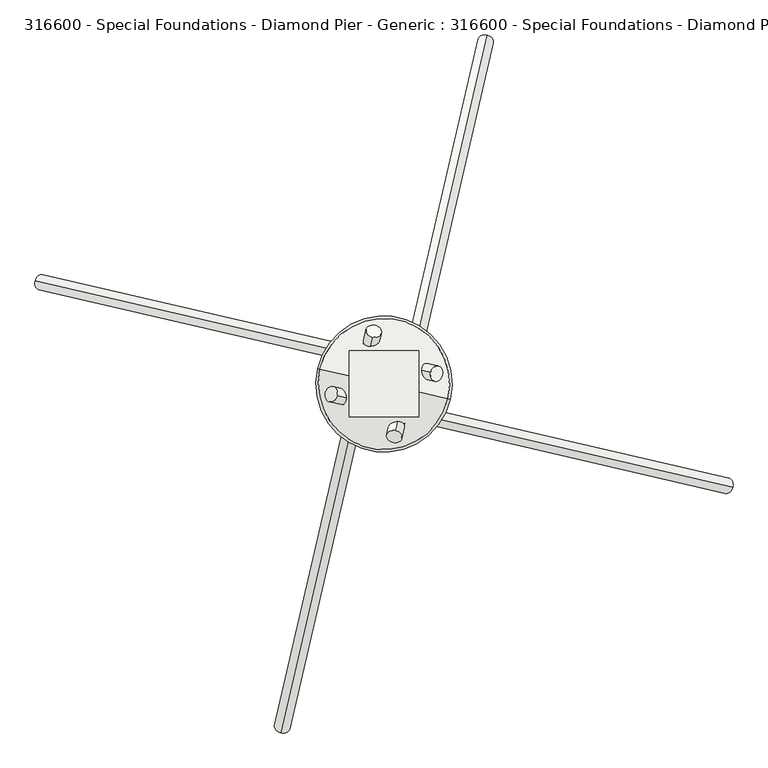
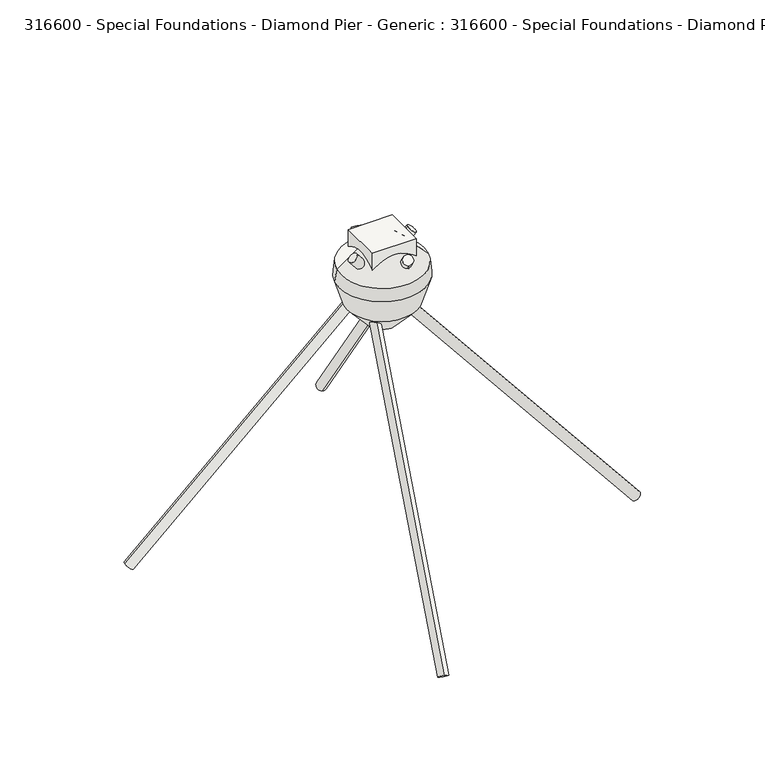
"""IFC4 building model written with IfcOpenShell, lengths in millimetres: slab geometry, 316600 - Special Foundations - Diamond Pier - Generic : 316600 - Special Foundations - Diamond Pier - Generic."""

from ifc_helpers import new_model, si_unit, point, frame, frame_2d, origin, place, context, project, spatial, polyline, circle_curve, trimmed, segment, composite_curve, outline, extrude, source, transform, mapped, element, save
from ifc_brep_helpers import plane_surface, revolved_surface, advanced_brep


def slab_316600_special_foundations_diamond_pier_generic_316600_ae65de88(model_context):
    return source(origin(), model_context, "Body", "SolidModel", [
        extrude(outline(composite_curve([segment(trimmed(circle_curve(frame_2d((1e-07, -15.875)), 15.875), [point((1e-07, -31.7500001))], [point((0.0, 0.0))], False, "CARTESIAN"), True, "CONTINUOUS"), segment(trimmed(circle_curve(frame_2d((1e-07, -15.875)), 15.875), [point((0.0, 0.0))], [point((1e-07, -31.7500001))], False, "CARTESIAN"), True, "CONTINUOUS")], self_intersect=False)), frame((-207.7929333, -703.2724242, -991.3584593), z_axis=(0.14520854647133766, 0.628002114484006, 0.7645441924671841), x_axis=(-0.9742942350214497, 0.2252792569322976, 0.0)), (0.0, 0.0, 1.0), 1270.0),
        extrude(outline(composite_curve([segment(trimmed(circle_curve(frame_2d((1e-07, -15.875)), 15.875), [point((1e-07, -31.7500001))], [point((0.0, 0.0))], False, "CARTESIAN"), True, "CONTINUOUS"), segment(trimmed(circle_curve(frame_2d((1e-07, -15.875)), 15.875), [point((0.0, 0.0))], [point((1e-07, -31.7500001))], False, "CARTESIAN"), True, "CONTINUOUS")], self_intersect=False)), frame((-703.2724242, 207.7929333, -991.3584593), z_axis=(0.6280021144840067, -0.14520854647133485, 0.7645441924671843), x_axis=(0.22527925693229323, 0.9742942350214507, 0.0)), (0.0, 0.0, 1.0), 1270.0),
        extrude(outline(composite_curve([segment(trimmed(circle_curve(frame_2d((1e-07, -15.875)), 15.875), [point((1e-07, -31.7500001))], [point((0.0, 0.0))], False, "CARTESIAN"), True, "CONTINUOUS"), segment(trimmed(circle_curve(frame_2d((1e-07, -15.875)), 15.875), [point((0.0, 0.0))], [point((1e-07, -31.7500001))], False, "CARTESIAN"), True, "CONTINUOUS")], self_intersect=False)), frame((207.7929333, 703.2724242, -991.3584593), z_axis=(-0.14520854647133596, -0.6280021144840063, 0.7645441924671844), x_axis=(0.9742942350214504, -0.22527925693229495, 0.0)), (0.0, 0.0, 1.0), 1270.0),
        extrude(outline(composite_curve([segment(trimmed(circle_curve(frame_2d((1e-07, -15.875)), 15.875), [point((1e-07, -31.7500001))], [point((0.0, 0.0))], False, "CARTESIAN"), True, "CONTINUOUS"), segment(trimmed(circle_curve(frame_2d((1e-07, -15.875)), 15.875), [point((0.0, 0.0))], [point((1e-07, -31.7500001))], False, "CARTESIAN"), True, "CONTINUOUS")], self_intersect=False)), frame((703.2724242, -207.7929333, -991.3584593), z_axis=(-0.6280021144840057, 0.14520854647133877, 0.7645441924671843), x_axis=(-0.22527925693229922, -0.9742942350214493, 0.0)), (0.0, 0.0, 1.0), 1270.0),
        advanced_brep(
        [(-108.3324504, 25.0489565, -217.3055075), (108.3324504, -25.0489565, -217.3055075), (42.5837569, -9.8463449, -291.7305661), (-42.5837569, 9.8463449, -291.7305661), (-133.8544614, 30.950233, -132.1736467), (133.8544614, -30.950233, -132.1736467), (-128.9734508, 29.821631, -90.9283538), (128.9734508, -29.821631, -90.9283538), (-48.2749795, 11.1622866, -12.7), (48.2749795, -11.1622866, -12.7), (0.0, 0.0, -12.7), (0.0, 0.0, -292.024192)],
        [
            (0, 1, circle_curve(frame((0.0, 0.0, -217.3055075), z_axis=(0.0, 0.0, -1.0), x_axis=(0.9742942350214493, -0.22527925693229933, 0.0)), 111.1906922)),
            (1, 2),
            (2, 3, circle_curve(frame((0.0, 0.0, -291.7305661), z_axis=(0.0, 0.0, 1.0), x_axis=(0.9742942350214493, -0.22527925693229933, 0.0)), 43.7072861)),
            (3, 0),
            (1, 0, circle_curve(frame((0.0, 0.0, -217.3055075), z_axis=(0.0, 0.0, -1.0), x_axis=(0.9742942350214493, -0.22527925693229933, 0.0)), 111.1906922)),
            (3, 2, circle_curve(frame((0.0, 0.0, -291.7305661), z_axis=(0.0, 0.0, 1.0), x_axis=(0.9742942350214493, -0.22527925693229933, 0.0)), 43.7072861)),
            (4, 5, circle_curve(frame((0.0, 0.0, -132.1736467), z_axis=(0.0, 0.0, -1.0), x_axis=(0.9742942350214493, -0.22527925693229933, 0.0)), 137.3860755)),
            (5, 1),
            (0, 4),
            (5, 4, circle_curve(frame((0.0, 0.0, -132.1736467), z_axis=(0.0, 0.0, -1.0), x_axis=(0.9742942350214493, -0.22527925693229933, 0.0)), 137.3860755)),
            (6, 7, circle_curve(frame((0.0, 0.0, -90.9283538), z_axis=(0.0, 0.0, -1.0), x_axis=(0.9742942350214493, -0.22527925693229933, 0.0)), 132.3762845)),
            (7, 5),
            (4, 6),
            (7, 6, circle_curve(frame((0.0, 0.0, -90.9283538), z_axis=(0.0, 0.0, -1.0), x_axis=(0.9742942350214493, -0.22527925693229933, 0.0)), 132.3762845)),
            (8, 9, circle_curve(frame((0.0, 0.0, -12.7), z_axis=(0.0, 0.0, -1.0), x_axis=(0.9742942350214493, -0.22527925693229933, 0.0)), 49.5486659)),
            (9, 7),
            (6, 8),
            (9, 8, circle_curve(frame((0.0, 0.0, -12.7), z_axis=(0.0, 0.0, -1.0), x_axis=(0.9742942350214493, -0.22527925693229933, 0.0)), 49.5486659)),
            (10, 9),
            (8, 10),
            (2, 11),
            (11, 3),
        ],
        [
            revolved_surface(polyline([(42.5837569, -9.8463449, -291.7305661), (108.3324504, -25.0489565, -217.3055075)]), (0.0, 0.0, -12.7), (0.0, 0.0, 1.0)),
            revolved_surface(polyline([(108.3324504, -25.0489565, -217.3055075), (133.8544614, -30.950233, -132.1736467)]), (0.0, 0.0, -12.7), (0.0, 0.0, 1.0)),
            revolved_surface(polyline([(133.8544614, -30.950233, -132.1736467), (128.9734508, -29.821631, -90.9283538)]), (0.0, 0.0, -12.7), (0.0, 0.0, 1.0)),
            revolved_surface(polyline([(128.9734508, -29.821631, -90.9283538), (48.2749795, -11.1622866, -12.7)]), (0.0, 0.0, -12.7), (0.0, 0.0, 1.0)),
            plane_surface(frame((0.0, 0.0, -12.7), z_axis=(0.0, 0.0, 1.0), x_axis=(0.9742942350214493, -0.22527925693229933, 0.0))),
            revolved_surface(polyline([(0.0, 0.0, -292.024192), (42.5837569, -9.8463449, -291.7305661)]), (0.0, 0.0, -12.7), (0.0, 0.0, 1.0)),
        ],
        [
            (0, [[1, 2, 3, 4]]),
            (0, [[5, -4, 6, -2]]),
            (1, [[7, 8, -1, 9]]),
            (1, [[10, -9, -5, -8]]),
            (2, [[11, 12, -7, 13]]),
            (2, [[14, -13, -10, -12]]),
            (3, [[15, 16, -11, 17]]),
            (3, [[18, -17, -14, -16]]),
            (4, [[19, -15, 20]]),
            (4, [[-20, -18, -19]]),
            (5, [[-3, 21, 22]]),
            (5, [[-6, -22, -21]]),
        ],
    ),
        extrude(outline(polyline([(70.369164, 66.5326915), (70.369164, -66.5326915), (-70.369164, -66.5326915), (-70.369164, 66.5326915), (70.369164, 66.5326915)])), frame((0.0, 0.0, -87.3372243), z_axis=(0.0, 0.0, 1.0), x_axis=(1.0, 0.0, 0.0)), (0.0, 0.0, 1.0), 87.3372243),
    ])


if __name__ == "__main__":
    model = new_model("IFC4")
    model_context = context("Model", 3, world=origin())
    ifc_project = project(units=[si_unit("LENGTHUNIT", "METRE", prefix="MILLI")], contexts=[model_context])
    site = spatial("IfcSite", under=ifc_project)
    building = spatial("IfcBuilding", under=site)
    placement = place(None, origin())
    slab_316600_special_foundations_diamond_pier_generic_316600_shape = slab_316600_special_foundations_diamond_pier_generic_316600_ae65de88(model_context)
    element("IfcSlab", 1, ObjectType="316600 - Special Foundations - Diamond Pier - Generic : 316600 - Special Foundations - Diamond Pier - Generic", at=placement, inside=building, context=model_context, shape_type="MappedRepresentation", body=[
        mapped(slab_316600_special_foundations_diamond_pier_generic_316600_shape, transform((0.0, 0.0, 0.0), x_axis=(1.0, 0.0, 0.0), y_axis=(0.0, 1.0, 0.0), z_axis=(0.0, 0.0, 1.0))),
    ])
    save(model, "model.ifc")

# Revit data of these elements
# Type "316600 - Special Foundations - Diamond Pier - Generic : 316600 - Special Foundations - Diamond Pier - Generic"
#   Assembly Code = "A1010100"
#   Structural Material = DIAMOND PIER DP-50/50 - (3300# B.L.C. AT 1500PSF SOILS, 4400# B.L.C. AT 2000PSF SOILS)
# Element 1 (IfcSlab, "316600 - Special Foundations - Diamond Pier - Generic : 316600 - Special Foundations - Diamond Pier - Generic")
#   Materials on its faces: "DIAMOND PIER DP-50/50 - (3300# B.L.C. AT 1500PSF SOILS, 4400# B.L.C. AT 2000PSF SOILS)"
# Materials
#   "DIAMOND PIER DP-50/50 - (3300# B.L.C. AT 1500PSF SOILS, 4400# B.L.C. AT 2000PSF SOILS)": class "Generic", colour RGB 195 195 195, transparency 0, Cost = 0
